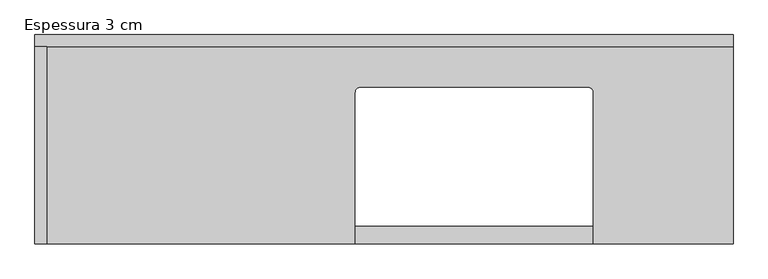
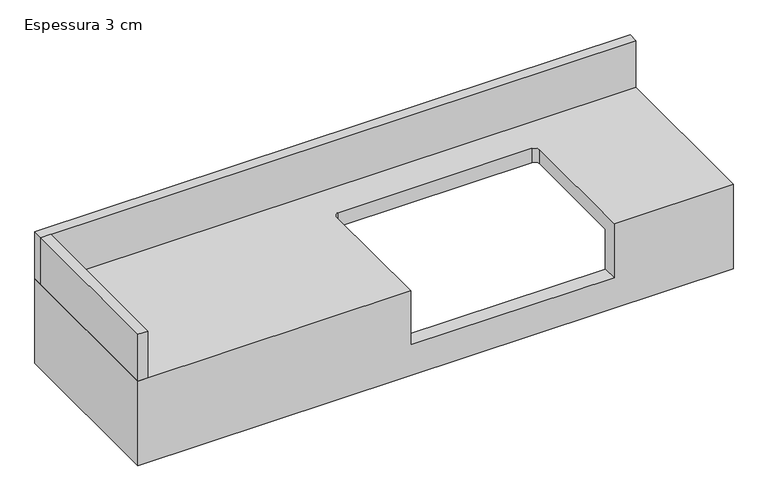
"""IFC4 building model written with IfcOpenShell, lengths in millimetres: furniture geometry, CC_BANCADA BANHEIRO COM CUBA_CANTO RETO : Espessura 3 cm."""

from ifc_helpers import new_model, si_unit, frame, origin, place, context, project, spatial, polyline, circle_curve, outline, extrude, source, transform, mapped, element, save
from ifc_brep_helpers import plane_surface, revolved_surface, advanced_brep


def espessura_3_cm_3b31cb49(model_context):
    return source(origin(), model_context, "Body", "SolidModel", [
        advanced_brep(
        [(750.0, 300.0, 860.0), (-450.0, 300.0, 860.0), (-450.0, -60.0, 860.0), (100.0, -60.0, 860.0), (100.0, 200.0, 860.0), (110.0, 210.0, 860.0), (500.0, 210.0, 860.0), (510.0, 200.0, 860.0), (510.0, -60.0, 860.0), (750.0, -60.0, 860.0), (750.0, 300.0, 680.0), (720.0, 300.0, 680.0), (720.0, 300.0, 830.0), (-420.0, 300.0, 830.0), (-420.0, 300.0, 680.0), (-450.0, 300.0, 680.0), (-450.0, -60.0, 680.0), (750.0, -60.0, 680.0), (510.0, -60.0, 745.0), (100.0, -60.0, 745.0), (720.0, -30.0, 830.0), (510.0, -30.0, 830.0), (510.0, 200.0, 830.0), (500.0, 210.0, 830.0), (110.0, 210.0, 830.0), (100.0, 200.0, 830.0), (100.0, -30.0, 830.0), (-420.0, -30.0, 830.0), (-420.0, -30.0, 680.0), (100.0, -30.0, 745.0), (510.0, -30.0, 745.0), (720.0, -30.0, 680.0)],
        [
            (0, 1),
            (1, 2),
            (2, 3),
            (3, 4),
            (4, 5, circle_curve(frame((110.0, 200.0, 860.0), z_axis=(0.0, 0.0, -1.0), x_axis=(0.0, 1.0, 0.0)), 10.0)),
            (5, 6),
            (6, 7, circle_curve(frame((500.0, 200.0, 860.0), z_axis=(0.0, 0.0, -1.0), x_axis=(0.0, 1.0, 0.0)), 10.0)),
            (7, 8),
            (8, 9),
            (9, 0),
            (0, 10),
            (10, 11),
            (11, 12),
            (12, 13),
            (13, 14),
            (14, 15),
            (15, 1),
            (15, 16),
            (16, 2),
            (16, 17),
            (17, 9),
            (8, 18),
            (18, 19),
            (19, 3),
            (17, 10),
            (12, 20),
            (20, 21),
            (21, 22),
            (22, 23, circle_curve(frame((500.0, 200.0, 830.0), z_axis=(0.0, 0.0, 1.0), x_axis=(0.0, 1.0, 0.0)), 10.0)),
            (23, 24),
            (24, 25, circle_curve(frame((110.0, 200.0, 830.0), z_axis=(0.0, 0.0, 1.0), x_axis=(0.0, 1.0, 0.0)), 10.0)),
            (25, 26),
            (26, 27),
            (27, 13),
            (27, 28),
            (28, 14),
            (26, 29),
            (29, 30),
            (30, 21),
            (20, 31),
            (31, 28),
            (11, 31),
            (5, 24),
            (23, 6),
            (18, 30),
            (29, 19),
            (4, 25),
            (7, 22),
        ],
        [
            plane_surface(frame((-450.0, 300.0, 860.0), z_axis=(0.0, 0.0, 1.0), x_axis=(-1.0, 0.0, 0.0))),
            plane_surface(frame((750.0, 300.0, 860.0), z_axis=(0.0, 1.0, 0.0), x_axis=(0.0, 0.0, -1.0))),
            plane_surface(frame((-450.0, 300.0, 860.0), z_axis=(-1.0, 0.0, 0.0), x_axis=(0.0, 0.0, -1.0))),
            plane_surface(frame((-450.0, -60.0, 860.0), z_axis=(0.0, -1.0, 0.0), x_axis=(0.0, 0.0, -1.0))),
            plane_surface(frame((750.0, -60.0, 860.0), z_axis=(1.0, 0.0, 0.0), x_axis=(0.0, 0.0, -1.0))),
            plane_surface(frame((-420.0, 300.0, 830.0), z_axis=(0.0, 0.0, -1.0), x_axis=(-1.0, 0.0, 0.0))),
            plane_surface(frame((-420.0, 300.0, 830.0), z_axis=(1.0, 0.0, 0.0), x_axis=(0.0, 0.0, -1.0))),
            plane_surface(frame((-420.0, -30.0, 830.0), z_axis=(0.0, 1.0, 0.0), x_axis=(0.0, 0.0, -1.0))),
            plane_surface(frame((720.0, -30.0, 830.0), z_axis=(-1.0, 0.0, 0.0), x_axis=(0.0, 0.0, -1.0))),
            plane_surface(frame((750.0, -60.0, 680.0), z_axis=(0.0, 0.0, -1.0), x_axis=(0.0, 1.0, 0.0))),
            plane_surface(frame((110.0, 210.0, 745.0), z_axis=(0.0, -1.0, 0.0), x_axis=(0.0, 0.0, 1.0))),
            plane_surface(frame((500.0, 210.0, 745.0), z_axis=(0.0, 0.0, 1.0), x_axis=(1.0, 0.0, 0.0))),
            revolved_surface(polyline([(110.0, 210.0, 830.0), (110.0, 210.0, 860.0)]), (110.0, 200.0, 900.0), (0.0, 0.0, -1.0)),
            plane_surface(frame((100.0, -190.0, 745.0), z_axis=(1.0, 0.0, 0.0), x_axis=(0.0, 0.0, 1.0))),
            plane_surface(frame((510.0, 200.0, 745.0), z_axis=(-1.0, 0.0, 0.0), x_axis=(0.0, 0.0, 1.0))),
            revolved_surface(polyline([(500.0, 210.0, 830.0), (500.0, 210.0, 860.0)]), (500.0, 200.0, 900.0), (0.0, 0.0, -1.0)),
        ],
        [
            (0, [[1, 2, 3, 4, 5, 6, 7, 8, 9, 10]]),
            (1, [[-1, 11, 12, 13, 14, 15, 16, 17]]),
            (2, [[-2, -17, 18, 19]]),
            (3, [[-3, -19, 20, 21, -9, 22, 23, 24]]),
            (4, [[-10, -21, 25, -11]]),
            (5, [[26, 27, 28, 29, 30, 31, 32, 33, 34, -14]]),
            (6, [[-34, 35, 36, -15]]),
            (7, [[-33, 37, 38, 39, -27, 40, 41, -35]]),
            (8, [[-26, -13, 42, -40]]),
            (9, [[-12, -25, -20, -18, -16, -36, -41, -42]]),
            (10, [[-6, 43, -30, 44]]),
            (11, [[-23, 45, -38, 46]]),
            (12, [[-5, 47, -31, -43]]),
            (13, [[-4, -24, -46, -37, -32, -47]]),
            (14, [[-8, 48, -28, -39, -45, -22]]),
            (15, [[-7, -44, -29, -48]]),
        ],
    ),
        extrude(outline(polyline([(-430.0, -60.0), (-450.0, -60.0), (-450.0, 280.0), (-430.0, 280.0), (-430.0, -60.0)])), frame((0.0, 0.0, 860.0), z_axis=(0.0, 0.0, 1.0), x_axis=(1.0, 0.0, 0.0)), (0.0, 0.0, 1.0), 100.0),
        extrude(outline(polyline([(750.0, 300.0), (750.0, 280.0), (-450.0, 280.0), (-450.0, 300.0), (750.0, 300.0)])), frame((0.0, 0.0, 860.0), z_axis=(0.0, 0.0, 1.0), x_axis=(1.0, 0.0, 0.0)), (0.0, 0.0, 1.0), 100.0),
    ])


if __name__ == "__main__":
    model = new_model("IFC4")
    model_context = context("Model", 3, world=origin())
    ifc_project = project(units=[si_unit("LENGTHUNIT", "METRE", prefix="MILLI")], contexts=[model_context])
    site = spatial("IfcSite", under=ifc_project)
    building = spatial("IfcBuilding", under=site)
    placement = place(None, origin())
    espessura_3_cm_shape = espessura_3_cm_3b31cb49(model_context)
    element("IfcFurniture", 1, ObjectType="CC_BANCADA BANHEIRO COM CUBA_CANTO RETO : Espessura 3 cm", at=placement, inside=building, context=model_context, shape_type="MappedRepresentation", body=[
        mapped(espessura_3_cm_shape, transform((0.0, 0.0, 0.0), x_axis=(1.0, 0.0, 0.0), y_axis=(0.0, 1.0, 0.0), z_axis=(0.0, 0.0, 1.0))),
    ])
    save(model, "model.ifc")

# Revit data of these elements
# Type "CC_BANCADA BANHEIRO COM CUBA_CANTO RETO : Espessura 3 cm"
#   Uso HS [instance default] = ""
#   h TESTEIRA AUX [instance default] = 0.15 m
#   Altura testeira [instance default] = 0.15 m
#   Altura rodapia [instance default] = 0.10 m
#   Espessura rodapia [instance default] = 0.02 m
#   Prof/2 [instance default] = 0.20 m
#   Offset cuba esquerda [instance default] = 0.40 m
#   Depth [instance default] = 1.20 m
#   Width [instance default] = 0.40 m
#   Espessura bancada = 0.03 m
#   Comprimento [instance default] = 1.20 m
#   Height [instance default] = 0.86 m
#   Testeira [instance default] = yes
#   Rodapia fundo [instance default] = no
#   Rodapia esquerda [instance default] = no
#   Rodapia direita [instance default] = no
#   Material porta-toalha [instance default] = .CROMADO
#   Material hidráulico [instance default] = .CROMADO
#   Material cuba [instance default] = .PORCELANA BRANCA
#   Material bancada [instance default] = .GRANITO_BRANCO_ITAUNAS
#   Assembly Code = ""
# Element 1 (IfcFurniture, "CC_BANCADA BANHEIRO COM CUBA_CANTO RETO : Espessura 3 cm")
#   Uso HS = "LAVABO"
#   Prof/2 = 0.18 m
#   Offset cuba esquerda = 0.55 m
#   Width = 0.36 m
#   Rodapia fundo = yes
#   Rodapia esquerda = yes
#   Materials on its faces: ".GRANITO_BRANCO_ITAUNAS"
# Materials
#   ".CROMADO": class "CC_METAIS", colour RGB 211 223 226, transparency 0, Cost = 0
#   ".PORCELANA BRANCA": class "CC_PORCELANA", colour RGB 230 230 230, transparency 0, Cost = 0
#   ".GRANITO_BRANCO_ITAUNAS": class ".CC_PEDRA REVEST.", colour RGB 202 195 174, transparency 0, Description = "Revestimento em granito", Cost = 0
